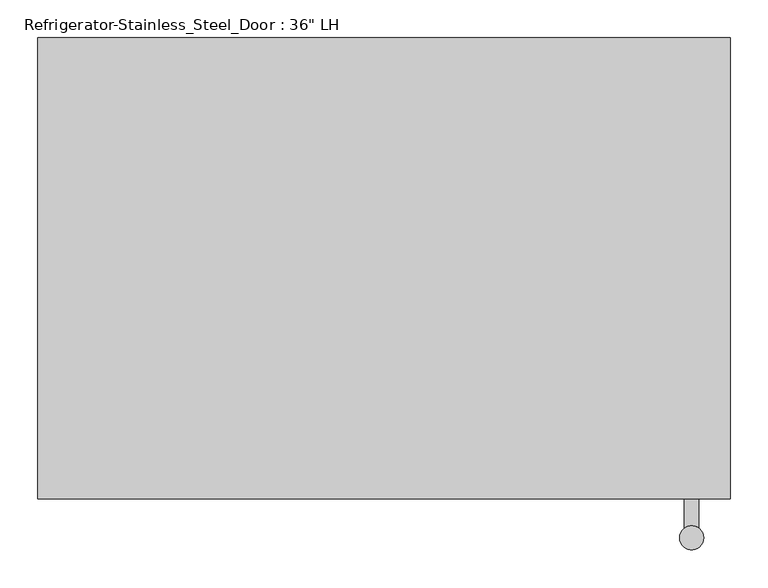
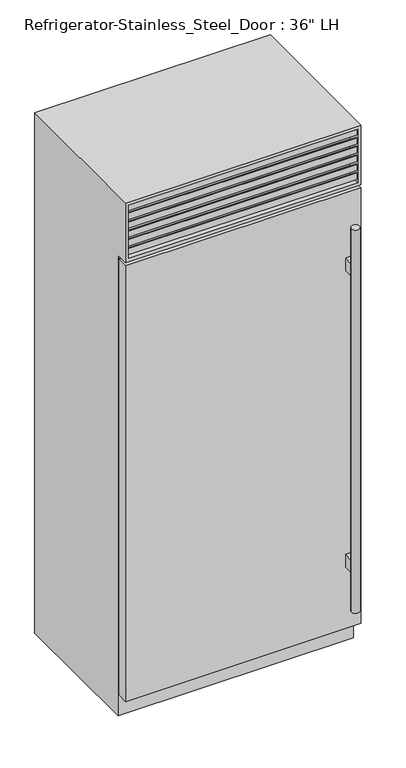
"""IFC4 building model written with IfcOpenShell, lengths in millimetres: proxy geometry."""

import ifcopenshell
import ifcopenshell.guid

model = None  # the IFC model being written
_history = None  # IfcOwnerHistory: only IFC2X3 demands one
_inside = {}  # id of a spatial element -> (the spatial element, [elements in it])
_under = {}  # id of a project, library or spatial element -> (it, [spatial elements below it])
_declared = {}  # id of a project -> (the project, [libraries it declares])
_typed = {}  # id of a type object -> (the type object, [elements of that type])
_made_of = {}  # id of a material, layer set ... -> (it, [elements and type objects made of it])


def new_model(schema):
    """Start an empty IFC model of exactly this schema.

    Asked for "IFC4X3", IfcOpenShell would pick the latest addendum, in which some entities
    have other attributes; the version numbers below select the first issue.
    IFC2X3 requires an IfcOwnerHistory on every rooted entity: one is made here for all.
    """
    global model, _history
    if schema == "IFC4X3":
        model = ifcopenshell.file(schema_version=(4, 3, 0, 0))
    else:
        model = ifcopenshell.file(schema=schema)
    _inside.clear()
    _under.clear()
    _declared.clear()
    _typed.clear()
    _made_of.clear()
    _history = None
    if model.schema == "IFC2X3":
        org = make("IfcOrganization", Name="unknown")
        user = make(
            "IfcPersonAndOrganization",
            ThePerson=make("IfcPerson", FamilyName="unknown"),
            TheOrganization=org,
        )
        app = make(
            "IfcApplication",
            ApplicationDeveloper=org,
            Version="unknown",
            ApplicationFullName="unknown",
            ApplicationIdentifier="unknown",
        )
        _history = make(
            "IfcOwnerHistory",
            OwningUser=user,
            OwningApplication=app,
            ChangeAction="ADDED",
            CreationDate=0,
        )
    return model


def make(cls, **values):
    """One entity of the class cls with the attributes given. An attribute that is None is left unset."""
    return model.create_entity(
        cls, **{name: value for name, value in values.items() if value is not None}
    )


def rooted(cls, **values):
    """An entity with a GlobalId (a new one), such as an element, a storey or a relation."""
    return make(cls, GlobalId=ifcopenshell.guid.new(), OwnerHistory=_history, **values)


def si_unit(unit_type, name, prefix=None):
    """IfcSIUnit, for example si_unit("LENGTHUNIT", "METRE", prefix="MILLI")."""
    return make("IfcSIUnit", UnitType=unit_type, Prefix=prefix, Name=name)


def assignment(units):
    """IfcUnitAssignment: the units of a project."""
    return None if units is None else make("IfcUnitAssignment", Units=units)


def point(xyz):
    """IfcCartesianPoint."""
    return None if xyz is None else make("IfcCartesianPoint", Coordinates=xyz)


def direction(xyz):
    """IfcDirection."""
    return None if xyz is None else make("IfcDirection", DirectionRatios=xyz)


def frame(location, z_axis=None, x_axis=None):
    """IfcAxis2Placement3D, a coordinate frame: its origin and axes. An axis left out is left unset."""
    return make(
        "IfcAxis2Placement3D",
        Location=point(location),
        Axis=direction(z_axis),
        RefDirection=direction(x_axis),
    )


def origin():
    """The frame at (0, 0, 0) with its axes left unset."""
    return frame((0.0, 0.0, 0.0))


def place(relative_to, where):
    """IfcLocalPlacement: puts the frame where relative to a parent placement (None: the world)."""
    return make(
        "IfcLocalPlacement", PlacementRelTo=relative_to, RelativePlacement=where
    )


def context(
    kind, dimensions, precision=None, world=None, true_north=None, identifier=None
):
    """IfcGeometricRepresentationContext, for example the 3D "Model" context."""
    return make(
        "IfcGeometricRepresentationContext",
        ContextIdentifier=identifier,
        ContextType=kind,
        CoordinateSpaceDimension=dimensions,
        Precision=precision,
        WorldCoordinateSystem=world,
        TrueNorth=true_north,
    )


def project(units=None, contexts=None):
    """IfcProject with its units and contexts."""
    return rooted(
        "IfcProject",
        Name="project",
        RepresentationContexts=contexts,
        UnitsInContext=assignment(units),
    )


def spatial(cls, under=None, at=None, **own):
    """A site, building, storey or space (cls), placed at a placement, below another one or the project."""
    s = rooted(cls, ObjectPlacement=at, **own)
    if under is not None:
        _under.setdefault(under.id(), (under, []))[1].append(s)
    return s


def polyline(points):
    """IfcPolyline through the points."""
    return make("IfcPolyline", Points=[point(p) for p in points])


def circle_curve(where, radius):
    """IfcCircle in the frame where."""
    return make("IfcCircle", Position=where, Radius=radius)


def ellipse_curve(where, semi_axis1, semi_axis2):
    """IfcEllipse in the frame where."""
    return make(
        "IfcEllipse", Position=where, SemiAxis1=semi_axis1, SemiAxis2=semi_axis2
    )


def outline(outer, holes=None, kind="AREA"):
    """IfcArbitraryClosedProfileDef: a profile drawn as a closed curve; with holes, ...WithVoids."""
    if holes is None:
        return make("IfcArbitraryClosedProfileDef", ProfileType=kind, OuterCurve=outer)
    return make(
        "IfcArbitraryProfileDefWithVoids",
        ProfileType=kind,
        OuterCurve=outer,
        InnerCurves=holes,
    )


def extrude(swept, where, along, depth):
    """IfcExtrudedAreaSolid: the profile swept, set in the frame where, extruded along a direction by depth."""
    return make(
        "IfcExtrudedAreaSolid",
        SweptArea=swept,
        Position=where,
        ExtrudedDirection=direction(along),
        Depth=depth,
    )


def faces_of(points, faces, orient=None, outer=None):
    """IfcFace entities. A face is a list of loops; a loop is a list of indices into points, from 0.

    orient and outer hold one flag for each loop. By default every Orientation is true, the
    first loop of a face is its IfcFaceOuterBound and the others are IfcFaceBound.
    """
    made = []
    for i, loops in enumerate(faces):
        bounds = []
        for j, loop in enumerate(loops):
            is_outer = j == 0 if outer is None else outer[i][j]
            bounds.append(
                make(
                    "IfcFaceOuterBound" if is_outer else "IfcFaceBound",
                    Bound=make("IfcPolyLoop", Polygon=[points[k] for k in loop]),
                    Orientation=True if orient is None else orient[i][j],
                )
            )
        made.append(make("IfcFace", Bounds=bounds))
    return made


def faceted_brep(points, faces, orient=None, outer=None, voids=None):
    """IfcFacetedBrep: a solid bounded by flat faces; with voids (closed shells), ...WithVoids."""
    shared = [point(p) for p in points]
    hull = make("IfcClosedShell", CfsFaces=faces_of(shared, faces, orient, outer))
    if voids is None:
        return make("IfcFacetedBrep", Outer=hull)
    return make(
        "IfcFacetedBrepWithVoids",
        Outer=hull,
        Voids=[
            make(cls, CfsFaces=faces_of(shared, fs, o, b)) for cls, fs, o, b in voids
        ],
    )


def shape(context_of_items, identifier, shape_type, items):
    """IfcShapeRepresentation: the items that make up one representation, for example the "Body"."""
    return make(
        "IfcShapeRepresentation",
        ContextOfItems=context_of_items,
        RepresentationIdentifier=identifier,
        RepresentationType=shape_type,
        Items=items,
    )


def source(mapping_origin, context_of_items, identifier, shape_type, items):
    """IfcRepresentationMap: a shape defined once, which mapped items show again and again."""
    return make(
        "IfcRepresentationMap",
        MappingOrigin=mapping_origin,
        MappedRepresentation=shape(context_of_items, identifier, shape_type, items),
    )


def transform(
    local_origin,
    x_axis=None,
    y_axis=None,
    z_axis=None,
    scale=None,
    scale2=None,
    scale3=None,
    uniform=True,
):
    """IfcCartesianTransformationOperator3D, or its non-uniform kind. x_axis, y_axis, z_axis: its Axis1, 2, 3."""
    if uniform:
        return make(
            "IfcCartesianTransformationOperator3D",
            Axis1=direction(x_axis),
            Axis2=direction(y_axis),
            LocalOrigin=point(local_origin),
            Scale=scale,
            Axis3=direction(z_axis),
        )
    return make(
        "IfcCartesianTransformationOperator3DnonUniform",
        Axis1=direction(x_axis),
        Axis2=direction(y_axis),
        LocalOrigin=point(local_origin),
        Scale=scale,
        Axis3=direction(z_axis),
        Scale2=scale2,
        Scale3=scale3,
    )


def mapped(mapping_source, mapping_target):
    """IfcMappedItem: shows the shape of a source again, moved by a transform."""
    return make(
        "IfcMappedItem", MappingSource=mapping_source, MappingTarget=mapping_target
    )


def made_of(thing, what):
    """Note that an element or type object is made of a material, layer set ...; save() writes the relation."""
    if what is not None:
        _made_of.setdefault(what.id(), (what, []))[1].append(thing)
    return thing


def element(
    cls,
    number,
    at=None,
    inside=None,
    cuts=None,
    type_object=None,
    material=None,
    context=None,
    identifier="Body",
    shape_type=None,
    held_by="IfcProductDefinitionShape",
    body=None,
    shapes=None,
    **own,
):
    """One element of the class cls, such as IfcWall. Its Tag is "e" and its number.

    at: its placement. inside: the storey or other place that contains it. cuts: it is an
    opening in that element (IfcRelVoidsElement). A single representation is given by context,
    identifier, shape_type and body (its items); several are given by shapes. held_by: the class
    of the entity that holds the representations. save() writes the other relations.
    """
    e = rooted(cls, Tag="e%d" % number, ObjectPlacement=at, **own)
    if body is not None:
        shapes = [shape(context, identifier, shape_type, body)]
    if shapes is not None:
        e.Representation = make(held_by, Representations=shapes)
    if inside is not None:
        _inside.setdefault(inside.id(), (inside, []))[1].append(e)
    if cuts is not None:
        rooted(
            "IfcRelVoidsElement", RelatingBuildingElement=cuts, RelatedOpeningElement=e
        )
    if type_object is not None:
        _typed.setdefault(type_object.id(), (type_object, []))[1].append(e)
    return made_of(e, material)


def aggregate(whole, parts):
    """IfcRelAggregates: a whole, such as a stair, and the parts it consists of."""
    return rooted("IfcRelAggregates", RelatingObject=whole, RelatedObjects=parts)


def save(model, path):
    """Write the relations noted so far, then the file.

    IfcRelAggregates (storeys below a building ...), IfcRelContainedInSpatialStructure (elements
    in a storey), IfcRelDefinesByType, IfcRelAssociatesMaterial and IfcRelDeclares: one each for
    every whole, place, type object, material and project.
    """
    for whole, parts in _under.values():
        aggregate(whole, parts)
    for where, things in _inside.values():
        rooted(
            "IfcRelContainedInSpatialStructure",
            RelatedElements=things,
            RelatingStructure=where,
        )
    for kind, things in _typed.values():
        rooted("IfcRelDefinesByType", RelatedObjects=things, RelatingType=kind)
    for what, things in _made_of.values():
        rooted("IfcRelAssociatesMaterial", RelatedObjects=things, RelatingMaterial=what)
    for by, libraries in _declared.values():
        rooted("IfcRelDeclares", RelatingContext=by, RelatedDefinitions=libraries)
    model.write(path)


def plane_surface(at):
    """IfcPlane: the flat surface through the origin of the frame at, square to its z axis."""
    return make("IfcPlane", Position=at)


def cylinder_surface(at, radius):
    """IfcCylindricalSurface: all points at the distance radius from the z axis of the frame at."""
    return make("IfcCylindricalSurface", Position=at, Radius=radius)


def advanced_brep(points, edges, surfaces, faces):
    """IfcAdvancedBrep: a solid bounded by faces that lie on surfaces and meet in shared edges.

    An edge is (start, end): straight between two places in points (the first is 0);
    or (start, end, curve); or (start, end, curve, False) where it runs against its curve.
    A face is (place in surfaces, loops), or (place, loops, False) where it looks against
    its surface's normal. A loop lists edges by number (the first is 1), with a minus sign
    where the edge is run from its end to its start. The first loop is the outer one.
    """
    corners = [point(p) for p in points]
    vertices = [make("IfcVertexPoint", VertexGeometry=c) for c in corners]
    made = []
    for start, end, *more in edges:
        made.append(
            make(
                "IfcEdgeCurve",
                EdgeStart=vertices[start],
                EdgeEnd=vertices[end],
                EdgeGeometry=more[0] if more else make("IfcPolyline", Points=[corners[start], corners[end]]),
                SameSense=more[1] if len(more) > 1 else True,
            )
        )
    hull = []
    for where, loops, *sense in faces:
        bounds = []
        for j, loop in enumerate(loops):
            ring = [make("IfcOrientedEdge", EdgeElement=made[abs(k) - 1], Orientation=k > 0) for k in loop]
            bounds.append(
                make(
                    "IfcFaceOuterBound" if j == 0 else "IfcFaceBound",
                    Bound=make("IfcEdgeLoop", EdgeList=ring),
                    Orientation=True,
                )
            )
        hull.append(make("IfcAdvancedFace", Bounds=bounds, FaceSurface=surfaces[where], SameSense=sense[0] if sense else True))
    return make("IfcAdvancedBrep", Outer=make("IfcClosedShell", CfsFaces=hull))


def proxy_425da594(model_context):
    return source(origin(), model_context, "Body", "SolidModel", [
        extrude(outline(polyline([(-457.2, -666.75), (457.2, -666.75), (457.2, -711.2), (-457.2, -711.2), (-457.2, -666.75)])), frame((0.0, 0.0, 88.9), z_axis=(0.0, 0.0, 1.0), x_axis=(1.0, 0.0, 0.0)), (0.0, 0.0, 1.0), 1787.525),
        faceted_brep([(457.2, -711.2, 2133.6), (-457.2, -711.2, 2133.6), (-457.2, -711.2, 1889.125), (457.2, -711.2, 1889.125), (444.5, -711.2, 2120.9), (444.5, -711.2, 1901.825), (-444.5, -711.2, 1901.825), (-444.5, -711.2, 2120.9), (457.2, -101.6, 2133.6), (-457.2, -101.6, 2133.6), (-457.2, -101.6, 0.0), (-457.2, -660.4, 0.0), (-457.2, -660.4, 1889.125), (457.2, -660.4, 1889.125), (457.2, -660.4, 0.0), (457.2, -101.6, 0.0), (-444.5, -660.4, 2120.9), (444.5, -660.4, 2120.9), (-444.5, -660.4, 1901.825), (444.5, -660.4, 1901.825)], [[[0, 1, 2, 3], [4, 5, 6, 7]], [[1, 0, 8, 9]], [[2, 1, 9, 10, 11, 12]], [[3, 2, 12, 13]], [[8, 0, 3, 13, 14, 15]], [[4, 7, 16, 17]], [[7, 6, 18, 16]], [[6, 5, 19, 18]], [[5, 4, 17, 19]], [[15, 14, 11, 10]], [[9, 8, 15, 10]], [[17, 16, 18, 19]], [[11, 14, 13, 12]]]),
        extrude(outline(polyline([(-660.4, 1901.825), (-708.025, 1914.5860803), (-708.025, 1939.9860803), (-704.85, 1939.9860803), (-704.85, 1917.1368938), (-660.4, 1905.2265522), (-660.4, 1901.825)])), frame((-444.5, 0.0, 0.0), z_axis=(1.0, 0.0, 0.0), x_axis=(0.0, 1.0, 0.0)), (0.0, 0.0, 1.0), 889.0),
        extrude(outline(polyline([(-660.4, 1938.0077839), (-708.025, 1950.7688642), (-708.025, 1976.1688642), (-704.85, 1976.1688642), (-704.85, 1953.3196777), (-660.4, 1941.4093361), (-660.4, 1938.0077839)])), frame((-444.5, 0.0, 0.0), z_axis=(1.0, 0.0, 0.0), x_axis=(0.0, 1.0, 0.0)), (0.0, 0.0, 1.0), 889.0),
        extrude(outline(polyline([(-660.4, 1974.1905679), (-708.025, 1986.9516482), (-708.025, 2012.3516482), (-704.85, 2012.3516482), (-704.85, 1989.5024616), (-660.4, 1977.59212), (-660.4, 1974.1905679)])), frame((-444.5, 0.0, 0.0), z_axis=(1.0, 0.0, 0.0), x_axis=(0.0, 1.0, 0.0)), (0.0, 0.0, 1.0), 889.0),
        extrude(outline(polyline([(-660.4, 2010.3733518), (-708.025, 2023.1344321), (-708.025, 2048.5344321), (-704.85, 2048.5344321), (-704.85, 2025.6852456), (-660.4, 2013.774904), (-660.4, 2010.3733518)])), frame((-444.5, 0.0, 0.0), z_axis=(1.0, 0.0, 0.0), x_axis=(0.0, 1.0, 0.0)), (0.0, 0.0, 1.0), 889.0),
        extrude(outline(polyline([(-660.4, 2046.5561358), (-708.025, 2059.3172161), (-708.025, 2084.7172161), (-704.85, 2084.7172161), (-704.85, 2061.8680295), (-660.4, 2049.9576879), (-660.4, 2046.5561358)])), frame((-444.5, 0.0, 0.0), z_axis=(1.0, 0.0, 0.0), x_axis=(0.0, 1.0, 0.0)), (0.0, 0.0, 1.0), 889.0),
        extrude(outline(polyline([(-660.4, 2082.7389197), (-708.025, 2095.5), (-708.025, 2120.9), (-704.85, 2120.9), (-704.85, 2098.0508135), (-660.4, 2086.1404719), (-660.4, 2082.7389197)])), frame((-444.5, 0.0, 0.0), z_axis=(1.0, 0.0, 0.0), x_axis=(0.0, 1.0, 0.0)), (0.0, 0.0, 1.0), 889.0),
        advanced_brep(
        [(-454.025, -666.75, 1873.25), (-454.025, -660.4, 1873.25), (-454.025, -660.4, 92.075), (-454.025, -666.75, 92.075), (-450.85, -660.4, 1870.075), (-450.85, -666.75, 1870.075), (-450.85, -666.75, 95.25), (-450.85, -660.4, 95.25), (454.025, -660.4, 92.075), (454.025, -666.75, 92.075), (450.85, -666.75, 95.25), (450.85, -660.4, 95.25), (454.025, -660.4, 1873.25), (454.025, -666.75, 1873.25), (450.85, -666.75, 1870.075), (450.85, -660.4, 1870.075)],
        [
            (0, 1, ellipse_curve(frame((-454.025, -663.575, 1873.25), z_axis=(-0.7071067811865474, 0.0, -0.7071067811865476), x_axis=(-0.7071067811865475, 0.0, 0.7071067811865475)), 4.4901281, 3.175)),
            (1, 2),
            (2, 3, ellipse_curve(frame((-454.025, -663.575, 92.075), z_axis=(-0.7071067811865476, 0.0, 0.7071067811865475), x_axis=(0.7071067811865474, 0.0, 0.7071067811865476)), 4.4901281, 3.175)),
            (3, 0),
            (4, 5),
            (5, 6),
            (6, 7),
            (7, 4),
            (2, 8),
            (8, 9, ellipse_curve(frame((454.025, -663.575, 92.075), z_axis=(-0.7071067811865475, 0.0, -0.7071067811865476), x_axis=(-0.7071067811865476, 0.0, 0.7071067811865474)), 4.4901281, 3.175)),
            (9, 3),
            (6, 10),
            (10, 11),
            (11, 7),
            (8, 12),
            (12, 13, ellipse_curve(frame((454.025, -663.575, 1873.25), z_axis=(0.7071067811865476, 0.0, -0.7071067811865475), x_axis=(-0.7071067811865474, 0.0, -0.7071067811865476)), 4.4901281, 3.175)),
            (13, 9),
            (10, 14),
            (14, 15),
            (15, 11),
            (1, 12),
            (15, 4),
            (0, 13),
            (5, 14),
        ],
        [
            cylinder_surface(frame((-454.025, -663.575, 1876.425), z_axis=(0.0, 0.0, 1.0), x_axis=(0.0, -1.0, 0.0)), 3.175),
            plane_surface(frame((-450.85, -666.75, 1870.075), z_axis=(1.0, 0.0, 0.0), x_axis=(0.0, 0.0, -1.0))),
            cylinder_surface(frame((-457.2, -663.575, 92.075), z_axis=(-1.0, 0.0, 0.0), x_axis=(0.0, -1.0, 0.0)), 3.175),
            plane_surface(frame((-450.85, -666.75, 95.25), z_axis=(0.0, 0.0, 1.0), x_axis=(1.0, 0.0, 0.0))),
            cylinder_surface(frame((454.025, -663.575, 88.9), z_axis=(0.0, 0.0, -1.0), x_axis=(0.0, -1.0, 0.0)), 3.175),
            plane_surface(frame((450.85, -666.75, 95.25), z_axis=(-1.0, 0.0, 0.0), x_axis=(0.0, 0.0, 1.0))),
            plane_surface(frame((450.85, -660.4, 1870.075), z_axis=(0.0, 1.0, 0.0), x_axis=(-1.0, 0.0, 0.0))),
            cylinder_surface(frame((457.2, -663.575, 1873.25), z_axis=(1.0, 0.0, 0.0), x_axis=(0.0, -1.0, 0.0)), 3.175),
            plane_surface(frame((454.025, -666.75, 1873.25), z_axis=(0.0, -1.0, 0.0), x_axis=(-1.0, 0.0, 0.0))),
            plane_surface(frame((450.85, -666.75, 1870.075), z_axis=(0.0, 0.0, -1.0), x_axis=(-1.0, 0.0, 0.0))),
        ],
        [
            (0, [[1, 2, 3, 4]]),
            (1, [[5, 6, 7, 8]]),
            (2, [[-3, 9, 10, 11]]),
            (3, [[-7, 12, 13, 14]]),
            (4, [[-10, 15, 16, 17]]),
            (5, [[-13, 18, 19, 20]]),
            (6, [[21, -15, -9, -2], [-14, -20, 22, -8]]),
            (7, [[-16, -21, -1, 23]]),
            (8, [[-11, -17, -23, -4], [24, -18, -12, -6]]),
            (9, [[-19, -24, -5, -22]]),
        ],
    ),
        advanced_brep(
        [(415.925, -711.2, 1609.725), (415.925, -711.2, 1558.925), (396.875, -711.2, 1558.925), (396.875, -711.2, 1609.725), (415.925, -711.2, 393.7), (415.925, -711.2, 342.9), (396.875, -711.2, 342.9), (396.875, -711.2, 393.7), (415.925, -749.6741958, 1609.725), (415.925, -749.6741958, 1558.925), (396.875, -749.6741958, 1558.925), (396.875, -749.6741958, 1609.725), (415.925, -749.6741958, 393.7), (415.925, -749.6741958, 342.9), (396.875, -749.6741958, 342.9), (396.875, -749.6741958, 393.7), (390.525, -762.3741958, 1762.125), (422.275, -762.3741958, 1762.125), (390.525, -762.3741958, 190.5), (422.275, -762.3741958, 190.5)],
        [
            (0, 1),
            (1, 2),
            (2, 3),
            (3, 0),
            (4, 5),
            (5, 6),
            (6, 7),
            (7, 4),
            (0, 8),
            (8, 9),
            (9, 1),
            (9, 10, circle_curve(frame((406.4, -762.3741958, 1558.925), z_axis=(0.0, 0.0, 1.0), x_axis=(1.0, 0.0, 0.0)), 15.875)),
            (10, 2),
            (10, 11),
            (11, 3),
            (11, 8, circle_curve(frame((406.4, -762.3741958, 1609.725), z_axis=(0.0, 0.0, -1.0), x_axis=(1.0, 0.0, 0.0)), 15.875)),
            (4, 12),
            (12, 13),
            (13, 5),
            (13, 14, circle_curve(frame((406.4, -762.3741958, 342.9), z_axis=(0.0, 0.0, 1.0), x_axis=(1.0, 0.0, 0.0)), 15.875)),
            (14, 6),
            (14, 15),
            (15, 7),
            (15, 12, circle_curve(frame((406.4, -762.3741958, 393.7), z_axis=(0.0, 0.0, -1.0), x_axis=(1.0, 0.0, 0.0)), 15.875)),
            (16, 17, circle_curve(frame((406.4, -762.3741958, 1762.125), z_axis=(0.0, 0.0, 1.0), x_axis=(1.0, 0.0, 0.0)), 15.875)),
            (17, 16, circle_curve(frame((406.4, -762.3741958, 1762.125), z_axis=(0.0, 0.0, 1.0), x_axis=(1.0, 0.0, 0.0)), 15.875)),
            (18, 19, circle_curve(frame((406.4, -762.3741958, 190.5), z_axis=(0.0, 0.0, -1.0), x_axis=(1.0, 0.0, 0.0)), 15.875)),
            (19, 18, circle_curve(frame((406.4, -762.3741958, 190.5), z_axis=(0.0, 0.0, -1.0), x_axis=(1.0, 0.0, 0.0)), 15.875)),
            (16, 18),
            (19, 17),
        ],
        [
            plane_surface(frame((415.925, -711.2, 1609.725), z_axis=(0.0, 1.0, 0.0), x_axis=(0.0, 0.0, -1.0))),
            plane_surface(frame((415.925, -711.2, 1609.725), z_axis=(1.0, 0.0, 0.0), x_axis=(0.0, -1.0, 0.0))),
            plane_surface(frame((415.925, -711.2, 1558.925), z_axis=(0.0, 0.0, -1.0), x_axis=(0.0, -1.0, 0.0))),
            plane_surface(frame((396.875, -711.2, 1558.925), z_axis=(-1.0, 0.0, 0.0), x_axis=(0.0, -1.0, 0.0))),
            plane_surface(frame((396.875, -711.2, 1609.725), z_axis=(0.0, 0.0, 1.0), x_axis=(0.0, -1.0, 0.0))),
            plane_surface(frame((415.925, -711.2, 393.7), z_axis=(1.0, 0.0, 0.0), x_axis=(0.0, -1.0, 0.0))),
            plane_surface(frame((415.925, -711.2, 342.9), z_axis=(0.0, 0.0, -1.0), x_axis=(0.0, -1.0, 0.0))),
            plane_surface(frame((396.875, -711.2, 342.9), z_axis=(-1.0, 0.0, 0.0), x_axis=(0.0, -1.0, 0.0))),
            plane_surface(frame((396.875, -711.2, 393.7), z_axis=(0.0, 0.0, 1.0), x_axis=(0.0, -1.0, 0.0))),
            plane_surface(frame((422.275, -762.3741958, 1762.125), z_axis=(0.0, 0.0, 1.0), x_axis=(0.0, 1.0, 0.0))),
            plane_surface(frame((422.275, -762.3741958, 190.5), z_axis=(0.0, 0.0, -1.0), x_axis=(0.0, -1.0, 0.0))),
            cylinder_surface(frame((406.4, -762.3741958, 190.5), z_axis=(0.0, 0.0, 1.0), x_axis=(1.0, 0.0, 0.0)), 15.875),
        ],
        [
            (0, [[1, 2, 3, 4]]),
            (0, [[5, 6, 7, 8]]),
            (1, [[-1, 9, 10, 11]]),
            (2, [[-2, -11, 12, 13]]),
            (3, [[-3, -13, 14, 15]]),
            (4, [[-4, -15, 16, -9]]),
            (5, [[-5, 17, 18, 19]]),
            (6, [[-6, -19, 20, 21]]),
            (7, [[-7, -21, 22, 23]]),
            (8, [[-8, -23, 24, -17]]),
            (9, [[25, 26]]),
            (10, [[27, 28]]),
            (11, [[-25, 29, -28, 30]]),
            (11, [[-26, -30, -27, -29], [-10, -16, -14, -12], [-18, -24, -22, -20]]),
        ],
    ),
    ])


if __name__ == "__main__":
    model = new_model("IFC4")
    model_context = context("Model", 3, world=origin())
    ifc_project = project(units=[si_unit("LENGTHUNIT", "METRE", prefix="MILLI")], contexts=[model_context])
    site = spatial("IfcSite", under=ifc_project)
    building = spatial("IfcBuilding", under=site)
    placement = place(None, origin())
    proxy_shape = proxy_425da594(model_context)
    element("IfcBuildingElementProxy", 1, Name="Refrigerator-Stainless_Steel_Door : 36\" LH", ObjectType="Refrigerator-Stainless_Steel_Door : 36\" LH", at=placement, inside=building, context=model_context, shape_type="MappedRepresentation", body=[
        mapped(proxy_shape, transform((0.0, 0.0, 0.0), x_axis=(1.0, 0.0, 0.0), y_axis=(0.0, 1.0, 0.0), z_axis=(0.0, 0.0, 1.0))),
    ])
    save(model, "model.ifc")

# Revit data of these elements
# Type "Refrigerator-Stainless_Steel_Door : 36\" LH"
#   Label = "Refrigerator"
#   Description = "Stainless Steel Door Refrigerator"
#   Assembly Code = "E1090320"
#   Width = 3' - 0"
#   Wall Offset = 0' - 4"
#   Voltage = 120 V
#   Power Consumption = 1000 VA
#   Height = 7' - 0"
#   Handle Centerline = 2' - 10"
#   Depth = 2' - 0"
#   Amperage = 8.33333 A
#   Show Label = yes
#   RH = no
#   LH = yes
#   Gasket = Appliance - Gasket
#   Appliance Finish = Appliance - Stainless Steel
#   Type Comments = ""
#   Default Elevation = 0
# Element 1 (IfcBuildingElementProxy, "Refrigerator-Stainless_Steel_Door : 36\" LH")
#   Materials on its faces: "Appliance - Stainless Steel", "Appliance - Gasket"
# Materials
#   "Appliance - Gasket": class "Miscellaneous", colour RGB 234 234 234, transparency 0, Cost = 0
#   "Appliance - Stainless Steel": class "Metal", colour RGB 189 187 185, transparency 0, Description = "Stainless Steel 18/8", Cost = 0
